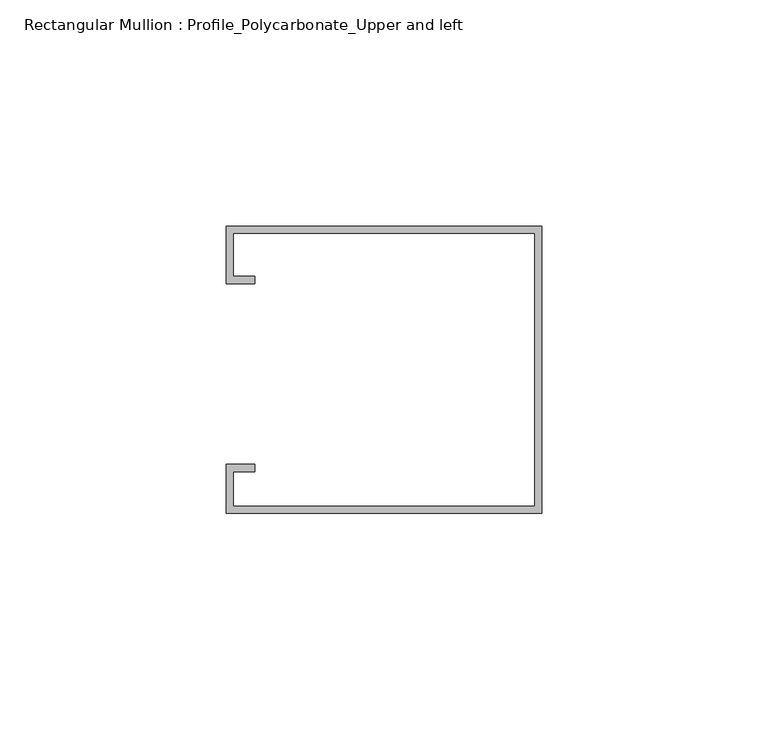
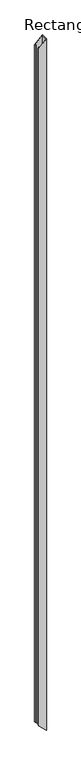
"""IFC4 building model written with IfcOpenShell, lengths in millimetres: member geometry, Rectangular Mullion : Profile_Polycarbonate_Upper and left."""

from ifc_helpers import new_model, si_unit, origin, place, context, project, spatial, faceted_brep, source, transform, mapped, element, save


def rectangular_mullion_profile_polycarbonate_upper_and_left_aec8978f(model_context):
    return source(origin(), model_context, "Body", "Brep", [
        faceted_brep([(-69.85, 32.7, -72.8210241), (0.0, 32.7, 0.0), (0.0, 32.7, -6695.5295347), (-69.85, 32.7, -6628.529344), (-69.85, 20.0, -72.8210241), (-69.85, 20.0, -6628.529344), (-63.5, 20.0, -66.200931), (-63.5, 20.0, -6634.6202704), (-63.5, 21.5875, -66.200931), (-63.5, 21.5875, -6634.6202704), (-68.2625, 21.5875, -71.1660008), (-68.2625, 21.5875, -6630.0520756), (-68.2625, 31.1125, -71.1660008), (-68.2625, 31.1125, -6630.0520756), (-1.5875, 31.1125, -1.6550233), (-1.5875, 31.1125, -6694.0068031), (-1.5875, -29.2125, -1.6550233), (-1.5875, -29.2125, -6694.0068031), (-68.2625, -29.2125, -71.1660008), (-68.2625, -29.2125, -6630.0520756), (-68.2625, -21.5875, -71.1660008), (-68.2625, -21.5875, -6630.0520756), (-63.5, -21.5875, -66.200931), (-63.5, -21.5875, -6634.6202704), (-63.5, -20.0, -66.200931), (-63.5, -20.0, -6634.6202704), (-69.85, -20.0, -72.8210241), (-69.85, -20.0, -6628.529344), (-69.85, -30.8, -72.8210241), (-69.85, -30.8, -6628.529344), (0.0, -30.8, 0.0), (0.0, -30.8, -6695.5295347)], [[[0, 1, 2, 3]], [[4, 0, 3, 5]], [[6, 4, 5, 7]], [[8, 6, 7, 9]], [[10, 8, 9, 11]], [[12, 10, 11, 13]], [[14, 12, 13, 15]], [[16, 14, 15, 17]], [[18, 16, 17, 19]], [[20, 18, 19, 21]], [[22, 20, 21, 23]], [[24, 22, 23, 25]], [[26, 24, 25, 27]], [[28, 26, 27, 29]], [[30, 28, 29, 31]], [[1, 30, 31, 2]], [[1, 0, 4, 6, 8, 10, 12, 14, 16, 18, 20, 22, 24, 26, 28, 30]], [[2, 31, 29, 27, 25, 23, 21, 19, 17, 15, 13, 11, 9, 7, 5, 3]]]),
    ])


if __name__ == "__main__":
    model = new_model("IFC4")
    model_context = context("Model", 3, world=origin())
    ifc_project = project(units=[si_unit("LENGTHUNIT", "METRE", prefix="MILLI")], contexts=[model_context])
    site = spatial("IfcSite", under=ifc_project)
    building = spatial("IfcBuilding", under=site)
    placement = place(None, origin())
    rectangular_mullion_profile_polycarbonate_upper_and_left_shape = rectangular_mullion_profile_polycarbonate_upper_and_left_aec8978f(model_context)
    element("IfcMember", 1, ObjectType="Rectangular Mullion : Profile_Polycarbonate_Upper and left", at=placement, inside=building, context=model_context, shape_type="MappedRepresentation", body=[
        mapped(rectangular_mullion_profile_polycarbonate_upper_and_left_shape, transform((0.0, 0.0, 0.0), x_axis=(1.0, 0.0, 0.0), y_axis=(0.0, 1.0, 0.0), z_axis=(0.0, 0.0, 1.0))),
    ])
    save(model, "model.ifc")

# Revit data of these elements
# Type "Rectangular Mullion : Profile_Polycarbonate_Upper and left"
#   built-in parameter 1007322 = 0.208333 (stored number, unit not read)
#   built-in parameter 1007321 = 0.00520833 (stored number, unit not read)
#   built-in parameter 1007320 = 0 (stored number, unit not read)
